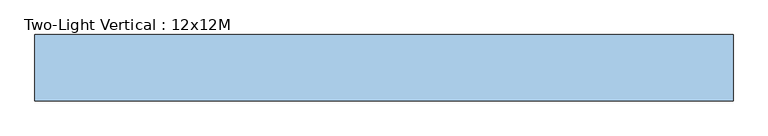
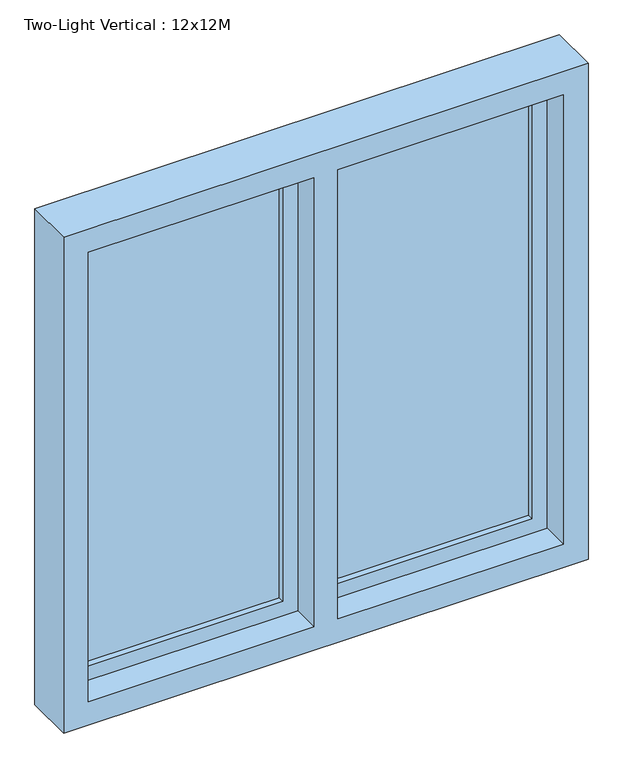
"""IFC4 building model written with IfcOpenShell, lengths in millimetres: window geometry, Two-Light Vertical : 12x12M."""

from ifc_helpers import new_model, si_unit, frame, origin, place, context, project, spatial, polyline, outline, extrude, faceted_brep, source, transform, mapped, element, save


def two_light_vertical_12x12m_7e3a313f(model_context):
    return source(origin(), model_context, "Body", "SolidModel", [
        extrude(outline(polyline([(1970.0, -624.0), (842.0, -624.0), (842.0, -72.5), (1970.0, -72.5), (1970.0, -624.0)]), holes=[polyline([(1920.0, -122.5), (892.0, -122.5), (892.0, -574.0), (1920.0, -574.0), (1920.0, -122.5)])]), frame((0.0, 134.0, 0.0), z_axis=(0.0, 1.0, 0.0), x_axis=(0.0, 0.0, 1.0)), (0.0, 0.0, 1.0), 50.0),
        extrude(outline(polyline([(1970.0, -47.5), (842.0, -47.5), (842.0, 504.0), (1970.0, 504.0), (1970.0, -47.5)]), holes=[polyline([(1920.0, 454.0), (892.0, 454.0), (892.0, 2.5), (1920.0, 2.5), (1920.0, 454.0)])]), frame((0.0, 134.0, 0.0), z_axis=(0.0, 1.0, 0.0), x_axis=(0.0, 0.0, 1.0)), (0.0, 0.0, 1.0), 50.0),
        faceted_brep([(-666.0, 184.0, 800.0), (546.0, 184.0, 800.0), (546.0, 69.0, 800.0), (-666.0, 69.0, 800.0), (546.0, 184.0, 2012.0), (546.0, 69.0, 2012.0), (-666.0, 184.0, 2012.0), (504.0, 184.0, 842.0), (504.0, 184.0, 1970.0), (-47.5, 184.0, 1970.0), (-47.5, 184.0, 842.0), (-624.0, 184.0, 842.0), (-72.5, 184.0, 842.0), (-72.5, 184.0, 1970.0), (-624.0, 184.0, 1970.0), (-666.0, 69.0, 2012.0), (489.0, 69.0, 1955.0), (489.0, 69.0, 857.0), (-32.5, 69.0, 857.0), (-32.5, 69.0, 1955.0), (-609.0, 69.0, 1955.0), (-87.5, 69.0, 1955.0), (-87.5, 69.0, 857.0), (-609.0, 69.0, 857.0), (489.0, 134.0, 857.0), (-32.5, 134.0, 857.0), (-609.0, 134.0, 857.0), (-87.5, 134.0, 857.0), (489.0, 134.0, 1955.0), (504.0, 134.0, 1970.0), (504.0, 134.0, 842.0), (-47.5, 134.0, 842.0), (-47.5, 134.0, 1970.0), (-32.5, 134.0, 1955.0), (-624.0, 134.0, 842.0), (-624.0, 134.0, 1970.0), (-72.5, 134.0, 1970.0), (-72.5, 134.0, 842.0), (-609.0, 134.0, 1955.0), (-87.5, 134.0, 1955.0)], [[[0, 1, 2, 3]], [[2, 1, 4, 5]], [[4, 1, 0, 6], [7, 8, 9, 10], [11, 12, 13, 14]], [[2, 5, 15, 3], [16, 17, 18, 19], [20, 21, 22, 23]], [[17, 24, 25, 18]], [[26, 23, 22, 27]], [[24, 17, 16, 28]], [[29, 30, 31, 32], [24, 28, 33, 25]], [[34, 35, 36, 37], [38, 26, 27, 39]], [[31, 30, 7, 10]], [[11, 34, 37, 12]], [[7, 30, 29, 8]], [[15, 6, 0, 3]], [[38, 20, 23, 26]], [[14, 35, 34, 11]], [[10, 9, 32, 31]], [[19, 18, 25, 33]], [[22, 21, 39, 27]], [[13, 12, 37, 36]], [[15, 5, 4, 6]], [[28, 16, 19, 33]], [[20, 38, 39, 21]], [[8, 29, 32, 9]], [[36, 35, 14, 13]]]),
        extrude(outline(polyline([(-574.0, 170.0), (-122.5, 170.0), (-122.5, 148.0), (-574.0, 148.0), (-574.0, 170.0)])), frame((0.0, 0.0, 892.0), z_axis=(0.0, 0.0, 1.0), x_axis=(1.0, 0.0, 0.0)), (0.0, 0.0, 1.0), 1028.0),
        extrude(outline(polyline([(2.5, 170.0), (454.0, 170.0), (454.0, 148.0), (2.5, 148.0), (2.5, 170.0)])), frame((0.0, 0.0, 892.0), z_axis=(0.0, 0.0, 1.0), x_axis=(1.0, 0.0, 0.0)), (0.0, 0.0, 1.0), 1028.0),
    ])


if __name__ == "__main__":
    model = new_model("IFC4")
    model_context = context("Model", 3, world=origin())
    ifc_project = project(units=[si_unit("LENGTHUNIT", "METRE", prefix="MILLI")], contexts=[model_context])
    site = spatial("IfcSite", under=ifc_project)
    building = spatial("IfcBuilding", under=site)
    placement = place(None, origin())
    two_light_vertical_12x12m_shape = two_light_vertical_12x12m_7e3a313f(model_context)
    element("IfcWindow", 1, ObjectType="Two-Light Vertical : 12x12M", at=placement, inside=building, context=model_context, shape_type="MappedRepresentation", body=[
        mapped(two_light_vertical_12x12m_shape, transform((0.0, 0.0, 0.0), x_axis=(1.0, 0.0, 0.0), y_axis=(0.0, 1.0, 0.0), z_axis=(0.0, 0.0, 1.0))),
    ])
    save(model, "model.ifc")

# Revit data of these elements
# Type "Two-Light Vertical : 12x12M"
#   Type Mark = "52"
#   Creator Organization [instance default] = "© Danish Educational Content"
#   Creator Name [instance default] = "© Erik Falck Jørgensen"
#   Creator Build [instance default] = "2017.0801.0"
#   Analytic Construction = "<None>"
#   length#5 = -36 mm
#   length#4 = -14 mm
#   length#3 = 120 mm
#   length#2 = 57 mm
#   length#1 = 0 mm
#   Seal Width = 12 mm
#   Rough Width = 1212 mm
#   Rough Height = 1212 mm
#   Rabbet Width = 15 mm
#   Rebate Depth = 50 mm
#   Transom Width = 55 mm
#   Rabbet Depth = 50 mm
#   Height = 1188 mm
#   Glass Thickness = 22 mm
#   Frame Width = 50 mm
#   Frame Depth = 50 mm
#   Exterior Direction [instance default] = 0.00°
#   Case Depth = 115 mm
#   Case Width = 45 mm
#   Default Sill Height = 800 mm
#   Width = 1188 mm
#   Sealing = no
#   Hinging = yes
#   Wall Closure = 1
#   Above Cutplane [instance default] = no
#   Glass = none
#   Case/Transom = none
#   Frame/Mullion = none
#   Assembly Code = ""
# Element 1 (IfcWindow, "Two-Light Vertical : 12x12M")
#   Materials on its faces: "Default Frame/Mullion (Interior/Exterior)", "Glass"
# Materials
#   "Default Frame/Mullion (Interior/Exterior)": class "Generic", colour RGB 205 205 205, transparency 0, Description = "Udefineret karm/ramme materiale", Cost = 0
#   "Glass": class "Glass", colour RGB 180 200 255, transparency 0.75, Description = "Generisk glas", Cost = 0
